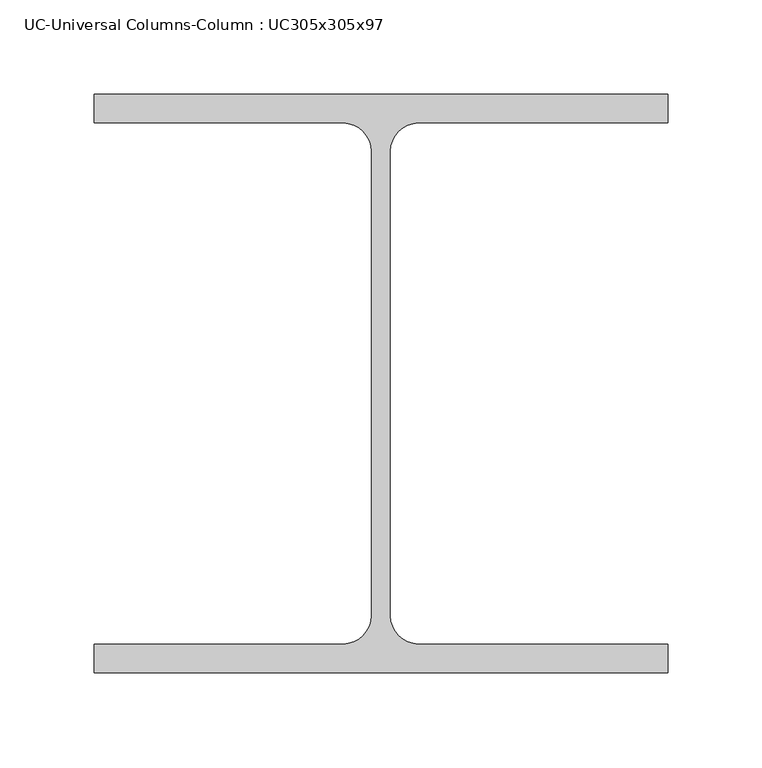
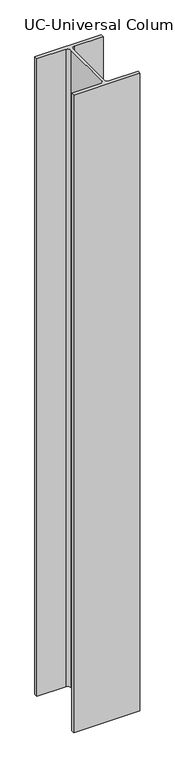
"""IFC4 building model written with IfcOpenShell, lengths in millimetres: column geometry, UC-Universal Columns-Column : UC305x305x97."""

from ifc_helpers import new_model, si_unit, point, frame, frame_2d, origin, place, context, project, spatial, polyline, circle_curve, trimmed, segment, composite_curve, outline, extrude, source, transform, mapped, element, save


def uc_universal_columns_column_uc305x305x97_b067ee91(model_context):
    return source(origin(), model_context, "Body", "SweptSolid", [
        extrude(outline(composite_curve([segment(polyline([(152.65, 153.95), (152.65, 138.55), (20.15, 138.55)]), True, "CONTINUOUS"), segment(trimmed(circle_curve(frame_2d((20.15, 123.35)), 15.2), [point((20.15, 138.55))], [point((4.95, 123.35))], True, "CARTESIAN"), True, "CONTINUOUS"), segment(polyline([(4.95, 123.35), (4.95, -123.35)]), True, "CONTINUOUS"), segment(trimmed(circle_curve(frame_2d((20.15, -123.35)), 15.2), [point((4.95, -123.35))], [point((20.15, -138.55))], True, "CARTESIAN"), True, "CONTINUOUS"), segment(polyline([(20.15, -138.55), (152.65, -138.55), (152.65, -153.95), (-152.65, -153.95), (-152.65, -138.55), (-20.15, -138.55)]), True, "CONTINUOUS"), segment(trimmed(circle_curve(frame_2d((-20.15, -123.35)), 15.2), [point((-20.15, -138.55))], [point((-4.95, -123.35))], True, "CARTESIAN"), True, "CONTINUOUS"), segment(polyline([(-4.95, -123.35), (-4.95, 123.35)]), True, "CONTINUOUS"), segment(trimmed(circle_curve(frame_2d((-20.15, 123.35)), 15.2), [point((-4.95, 123.35))], [point((-20.15, 138.55))], True, "CARTESIAN"), True, "CONTINUOUS"), segment(polyline([(-20.15, 138.55), (-152.65, 138.55), (-152.65, 153.95), (152.65, 153.95)]), True, "CONTINUOUS")], self_intersect=False)), frame((0.0, 0.0, 2900.0), z_axis=(0.0, 0.0, 1.0), x_axis=(1.0, 0.0, 0.0)), (0.0, 0.0, 1.0), 3100.0),
    ])


if __name__ == "__main__":
    model = new_model("IFC4")
    model_context = context("Model", 3, world=origin())
    ifc_project = project(units=[si_unit("LENGTHUNIT", "METRE", prefix="MILLI")], contexts=[model_context])
    site = spatial("IfcSite", under=ifc_project)
    building = spatial("IfcBuilding", under=site)
    placement = place(None, origin())
    uc_universal_columns_column_uc305x305x97_shape = uc_universal_columns_column_uc305x305x97_b067ee91(model_context)
    element("IfcColumn", 1, ObjectType="UC-Universal Columns-Column : UC305x305x97", at=placement, inside=building, context=model_context, shape_type="MappedRepresentation", body=[
        mapped(uc_universal_columns_column_uc305x305x97_shape, transform((0.0, 0.0, 0.0), x_axis=(1.0, 0.0, 0.0), y_axis=(0.0, 1.0, 0.0), z_axis=(0.0, 0.0, 1.0))),
    ])
    save(model, "model.ifc")

# Revit data of these elements
# Type "UC-Universal Columns-Column : UC305x305x97"
#   Section Name Key = "UC305x305x97"
#   Cost = 2
#   Width = 30.53 cm
#   Web Thickness = 0.99 cm
#   Web Fillet = 1.52 cm
#   Warping Constant = 1560000.0 cm⁶
#   Torsional Moment of Inertia = 91.20 cm⁴
#   Section Area = 123.0 cm²
#   Plastic Modulus weak axis = 726.0 cm³
#   Plastic Modulus strong axis = 1592.0 cm³
#   Nominal Weight = 96.8996 kgf/m
#   Moment of Inertia weak axis = 7308.00 cm⁴
#   Moment of Inertia strong axis = 22249.00 cm⁴
#   Height = 30.79 cm
#   Flange Thickness = 1.54 cm
#   Elastic Modulus weak axis = 479.0 cm³
#   Elastic Modulus strong axis = 1445.0 cm³
#   Centroid Vertical = 15.395 cm
#   Centroid Horizontal = 15.265 cm
#   Bolt Spacing = 14.0 cm
#   Structural Material [instance default] = Metal - Steel 43-275
#   Type Comments = ""
#   Assembly Code = ""
# Element 1 (IfcColumn, "UC-Universal Columns-Column : UC305x305x97")
#   Materials on its faces: "Metal - Steel 43-275"
# Materials
#   "Metal - Steel 43-275": class "Metal", colour RGB 247 247 247, transparency 0, Cost = 0
